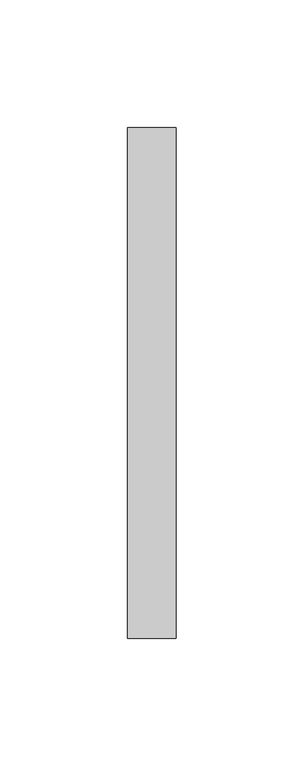
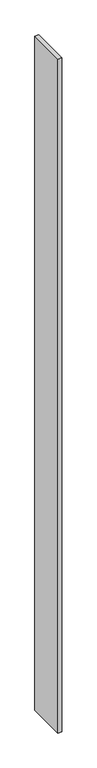
"""IFC4 building model written with IfcOpenShell, lengths in millimetres: proxy geometry, Inner panel:Inner panel:1:Inner panel:1 : Inner panel:Inner panel:300324:300043:Inner panel:1:Inner panel:1 : Inner panel:Inner panel:300324:300043 : Inner panel:Inner panel:1:Inner panel:1 : Inner panel:Inner panel:300324:300043:3 : Inner panel:Inner panel:1:Inner panel:1 : Inner panel:Inner panel:300324:300043:Inner panel:1:Inner panel:1 : Inner panel:Inner panel:300324:300043 : Inner panel:Inner panel:1:Inner panel:1 : Inner panel:Inner panel:300324:300043:300031."""

from ifc_helpers import new_model, si_unit, frame, origin, place, context, project, spatial, polyline, outline, extrude, source, transform, mapped, element, save


def generic_models_162e9f92(model_context):
    return source(origin(), model_context, "Body", "SweptSolid", [
        extrude(outline(polyline([(593719.0367239, -578797.4913841), (593738.0867239, -578797.4913841), (593738.0867239, -578997.5163841), (593719.0367239, -578997.5163841), (593719.0367239, -578797.4913841)])), frame((0.0, 0.0, 44.45), z_axis=(0.0, 0.0, 1.0), x_axis=(1.0, 0.0, 0.0)), (0.0, 0.0, 1.0), 3570.1761997),
    ])


if __name__ == "__main__":
    model = new_model("IFC4")
    model_context = context("Model", 3, world=origin())
    ifc_project = project(units=[si_unit("LENGTHUNIT", "METRE", prefix="MILLI")], contexts=[model_context])
    site = spatial("IfcSite", under=ifc_project)
    building = spatial("IfcBuilding", under=site)
    placement = place(None, origin())
    generic_models_shape = generic_models_162e9f92(model_context)
    element("IfcBuildingElementProxy", 1, Name="Inner panel:Inner panel:1:Inner panel:1 : Inner panel:Inner panel:300324:300043:Inner panel:1:Inner panel:1 : Inner panel:Inner panel:300324:300043 : Inner panel:Inner panel:1:Inner panel:1 : Inner panel:Inner panel:300324:300043:3 : Inner panel:Inner panel:1:Inner panel:1 : Inner panel:Inner panel:300324:300043:Inner panel:1:Inner panel:1 : Inner panel:Inner panel:300324:300043 : Inner panel:Inner panel:1:Inner panel:1 : Inner panel:Inner panel:300324:300043:300031", ObjectType="Inner panel:Inner panel:1:Inner panel:1 : Inner panel:Inner panel:300324:300043:Inner panel:1:Inner panel:1 : Inner panel:Inner panel:300324:300043 : Inner panel:Inner panel:1:Inner panel:1 : Inner panel:Inner panel:300324:300043:3 : Inner panel:Inner panel:1:Inner panel:1 : Inner panel:Inner panel:300324:300043:Inner panel:1:Inner panel:1 : Inner panel:Inner panel:300324:300043 : Inner panel:Inner panel:1:Inner panel:1 : Inner panel:Inner panel:300324:300043:300031", at=placement, inside=building, context=model_context, shape_type="MappedRepresentation", body=[
        mapped(generic_models_shape, transform((0.0, 0.0, 0.0), x_axis=(1.0, 0.0, 0.0), y_axis=(0.0, 1.0, 0.0), z_axis=(0.0, 0.0, 1.0))),
    ])
    save(model, "model.ifc")

# Revit data of these elements
# Type "Inner panel:Inner panel:1:Inner panel:1 : Inner panel:Inner panel:300324:300043:Inner panel:1:Inner panel:1 : Inner panel:Inner panel:300324:300043 : Inner panel:Inner panel:1:Inner panel:1 : Inner panel:Inner panel:300324:300043:3 : Inner panel:Inner panel:1:Inner panel:1 : Inner panel:Inner panel:300324:300043:Inner panel:1:Inner panel:1 : Inner panel:Inner panel:300324:300043 : Inner panel:Inner panel:1:Inner panel:1 : Inner panel:Inner panel:300324:300043:300031"
#   NameOverride = "Inner panel:Inner panel:1:Inner panel:1 : Inner panel:Inner panel:300324:300043:Inner panel:1:Inner panel:1 : Inner panel:Inner panel:300324:300043 : Inner panel:Inner panel:1:Inner panel:1 : Inner panel:Inner panel:300324:300043:300031"
#   ObjectTypeOverride = "Inner panel:1:Inner panel:1 : Inner panel:Inner panel:300324:300043 : Inner panel:Inner panel:1:Inner panel:1 : Inner panel:Inner panel:300324:300043"
#   Reference = "Inner panel"
#   Tag = "300031"
# Element 1 (IfcBuildingElementProxy, "Inner panel:Inner panel:1:Inner panel:1 : Inner panel:Inner panel:300324:300043:Inner panel:1:Inner panel:1 : Inner panel:Inner panel:300324:300043 : Inner panel:Inner panel:1:Inner panel:1 : Inner panel:Inner panel:300324:300043:3 : Inner panel:Inner panel:1:Inner panel:1 : Inner panel:Inner panel:300324:300043:Inner panel:1:Inner panel:1 : Inner panel:Inner panel:300324:300043 : Inner panel:Inner panel:1:Inner panel:1 : Inner panel:Inner panel:300324:300043:300031")
#   Materials on its faces: "¾” (CLASS A) FIRE RETARDANT PLYWOOD ...OR… IF 1/4\" GYP. BD UNDER PLYWOOD, FLAME SPREAD TO BE CLASS C -  (FINISH: GRADE B - PREFINISHED STAINED/SEALED) - 1/4\" GAP BTWN PANELS (FASTENERS T.B.D.)"
# Materials
#   "¾” (CLASS A) FIRE RETARDANT PLYWOOD ...OR… IF 1/4\" GYP. BD UNDER PLYWOOD, FLAME SPREAD TO BE CLASS C -  (FINISH: GRADE B - PREFINISHED STAINED/SEALED) - 1/4\" GAP BTWN PANELS (FASTENERS T.B.D.)": class "Wood", colour RGB 149 120 74, transparency 0, Description = "Plywood, sheathing grade", Cost = 0
